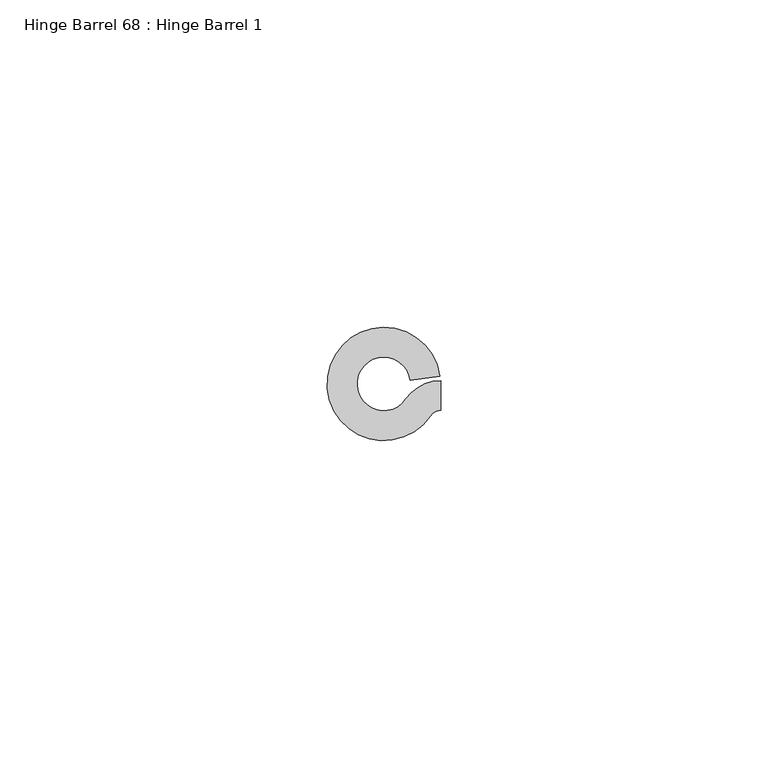
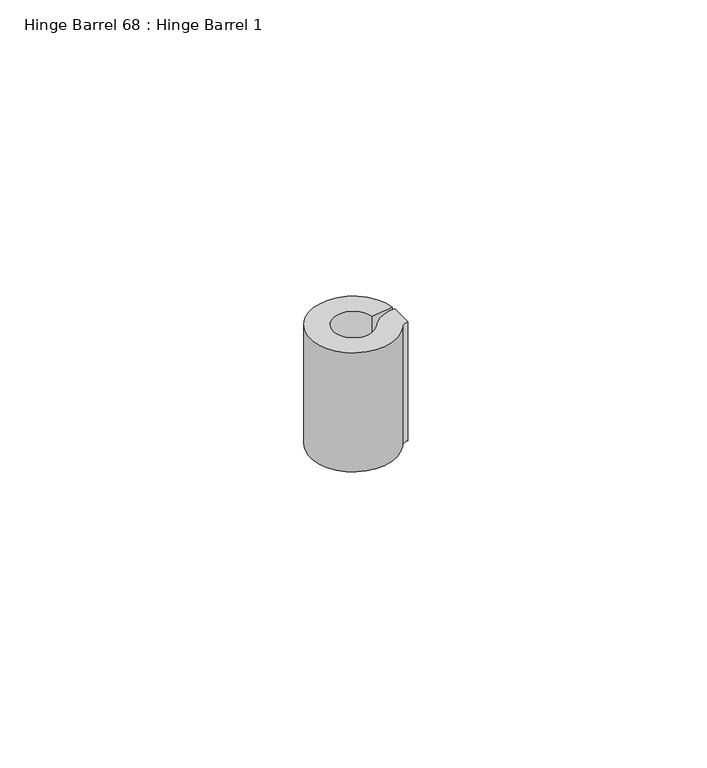
"""IFC4 building model written with IfcOpenShell, lengths in millimetres: proxy geometry, Hinge Barrel 68 : Hinge Barrel 1."""

from ifc_helpers import new_model, si_unit, point, frame, frame_2d, origin, place, context, project, spatial, polyline, circle_curve, trimmed, segment, composite_curve, outline, extrude, source, transform, mapped, element, save


def hinge_barrel_68_hinge_barrel_1_53ebecfd(model_context):
    return source(origin(), model_context, "Body", "SweptSolid", [
        extrude(outline(composite_curve([segment(trimmed(circle_curve(frame_2d((587327.8245257, -536316.2443067)), 6.4044851), [point((587322.5194669, -536312.6563017))], [point((587327.8245257, -536309.8398216))], False, "CARTESIAN"), True, "CONTINUOUS"), segment(polyline([(587327.8245257, -536309.8398216), (587327.8245257, -536314.4038841)]), True, "CONTINUOUS"), segment(trimmed(circle_curve(frame_2d((587327.8245257, -536316.2443067)), 1.8404226), [point((587327.8245257, -536314.4038841))], [point((587326.3000393, -536315.2132409))], True, "CARTESIAN"), True, "CONTINUOUS"), segment(trimmed(circle_curve(frame_2d((587319.1320739, -536310.3652841)), 8.6534625), [point((587326.3000393, -536315.2132409))], [point((587327.7022899, -536309.1678654))], False, "CARTESIAN"), True, "CONTINUOUS"), segment(polyline([(587327.7022899, -536309.1678654), (587323.1821338, -536309.7994153)]), True, "CONTINUOUS"), segment(trimmed(circle_curve(frame_2d((587319.1320739, -536310.3652841)), 4.0894), [point((587323.1821338, -536309.7994153))], [point((587322.5194669, -536312.6563017))], True, "CARTESIAN"), True, "CONTINUOUS")], self_intersect=False)), frame((0.0, 0.0, 1149.35), z_axis=(0.0, 0.0, 1.0), x_axis=(1.0, 0.0, 0.0)), (0.0, 0.0, 1.0), 25.4),
    ])


if __name__ == "__main__":
    model = new_model("IFC4")
    model_context = context("Model", 3, world=origin())
    ifc_project = project(units=[si_unit("LENGTHUNIT", "METRE", prefix="MILLI")], contexts=[model_context])
    site = spatial("IfcSite", under=ifc_project)
    building = spatial("IfcBuilding", under=site)
    placement = place(None, origin())
    hinge_barrel_68_hinge_barrel_1_shape = hinge_barrel_68_hinge_barrel_1_53ebecfd(model_context)
    element("IfcBuildingElementProxy", 1, Name="Hinge Barrel 68 : Hinge Barrel 1", ObjectType="Hinge Barrel 68 : Hinge Barrel 1", at=placement, inside=building, context=model_context, shape_type="MappedRepresentation", body=[
        mapped(hinge_barrel_68_hinge_barrel_1_shape, transform((0.0, 0.0, 0.0), x_axis=(1.0, 0.0, 0.0), y_axis=(0.0, 1.0, 0.0), z_axis=(0.0, 0.0, 1.0))),
    ])
    save(model, "model.ifc")

# Revit data of these elements
# Element 1 (IfcBuildingElementProxy, "Hinge Barrel 68 : Hinge Barrel 1")
#   Materials on its faces: "6\"X6\" WELD-ON STL BUTT HINGE"
# Materials
#   "6\"X6\" WELD-ON STL BUTT HINGE": class "Metal", colour RGB 189 187 185, transparency 0, Description = "Carbon steel", Cost = 0
